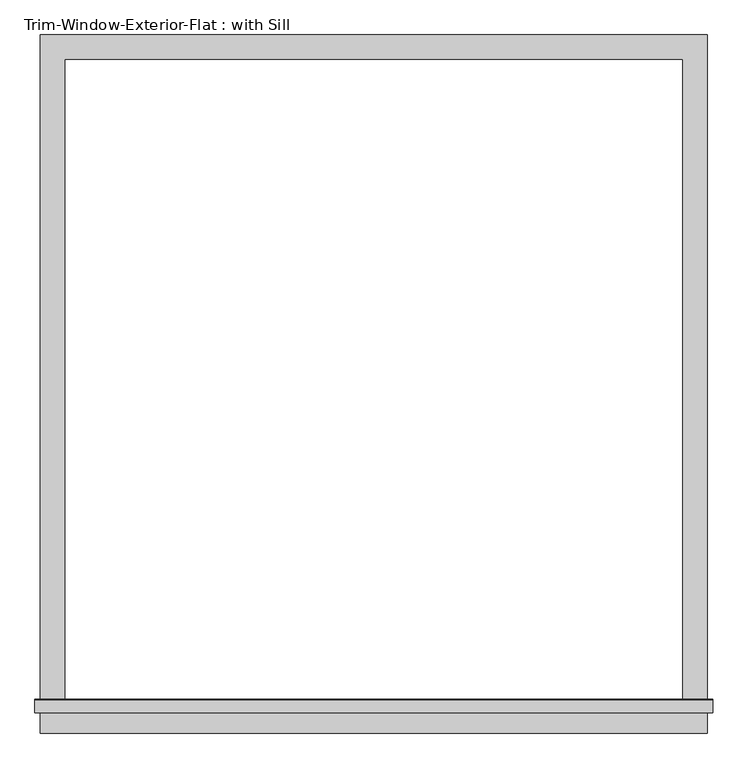
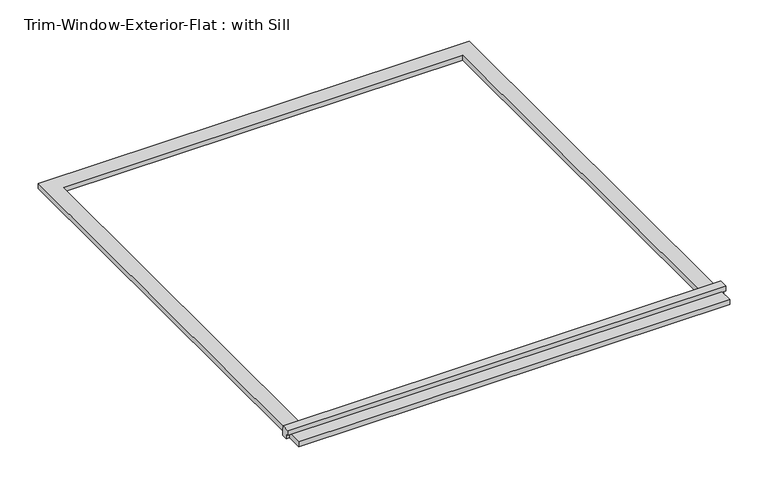
"""IFC4 building model written with IfcOpenShell, lengths in millimetres: proxy geometry, Trim-Window-Exterior-Flat : with Sill."""

from ifc_helpers import new_model, si_unit, frame, origin, origin_with_axes, place, context, project, spatial, polyline, outline, extrude, source, transform, mapped, element, save


def trim_window_exterior_flat_with_sill_b4b885c6(model_context):
    return source(origin(), model_context, "Body", "SweptSolid", [
        extrude(outline(polyline([(781.05, -1520.7823709), (781.05, -1577.9323709), (-781.05, -1577.9323709), (-781.05, -1520.7823709), (781.05, -1520.7823709)])), origin_with_axes(), (0.0, 0.0, 1.0), 19.05),
        extrude(outline(polyline([(-1530.35, 38.1), (-1501.0580645, 38.1), (-1498.6, 19.05), (-1498.6, 0.0), (-1520.7823709, 0.0), (-1520.7823709, 19.05), (-1530.35, 19.05), (-1530.35, 38.1)])), frame((-793.75, 0.0, 0.0), z_axis=(1.0, 0.0, 0.0), x_axis=(0.0, 1.0, 0.0)), (0.0, 0.0, 1.0), 1587.5),
        extrude(outline(polyline([(-781.05, 57.15), (781.05, 57.15), (781.05, -1498.6), (723.9, -1498.6), (723.9, 0.0), (-723.9, 0.0), (-723.9, -1498.6), (-781.05, -1498.6), (-781.05, 57.15)])), origin_with_axes(), (0.0, 0.0, 1.0), 19.05),
    ])


if __name__ == "__main__":
    model = new_model("IFC4")
    model_context = context("Model", 3, world=origin())
    ifc_project = project(units=[si_unit("LENGTHUNIT", "METRE", prefix="MILLI")], contexts=[model_context])
    site = spatial("IfcSite", under=ifc_project)
    building = spatial("IfcBuilding", under=site)
    placement = place(None, origin())
    trim_window_exterior_flat_with_sill_shape = trim_window_exterior_flat_with_sill_b4b885c6(model_context)
    element("IfcBuildingElementProxy", 1, Name="Trim-Window-Exterior-Flat : with Sill", ObjectType="Trim-Window-Exterior-Flat : with Sill", at=placement, inside=building, context=model_context, shape_type="MappedRepresentation", body=[
        mapped(trim_window_exterior_flat_with_sill_shape, transform((0.0, 0.0, 0.0), x_axis=(1.0, 0.0, 0.0), y_axis=(0.0, 1.0, 0.0), z_axis=(0.0, 0.0, 1.0))),
    ])
    save(model, "model.ifc")

# Revit data of these elements
# Type "Trim-Window-Exterior-Flat : with Sill"
#   Trim Width = 0' - 2 1/4"
#   Trim Thickness_Picture Frame = 0' - 1 1/4"
#   Trim Thickness_with Sill = 0' - 0 3/4"
#   Sill Thickness = 0' - 1 1/4"
#   Opening Width [instance default] = 2' - 0"
#   Opening Height [instance default] = 3' - 0"
#   Default Elevation = 4' - 0"
#   Sill = yes
#   Picture Frame = no
#   Trim Material [instance default] = none
# Element 1 (IfcBuildingElementProxy, "Trim-Window-Exterior-Flat : with Sill")
#   Opening Width = 4' - 9"
#   Opening Height = 4' - 11"
#   Trim Material = Clad - White
#   Materials on its faces: "Clad - White"
# Materials
#   "Clad - White": class "Wood", colour RGB 242 242 238, transparency 0, Cost = 0
